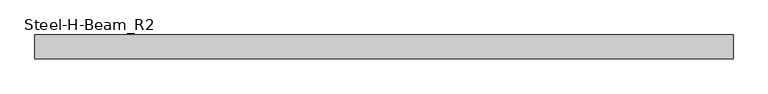
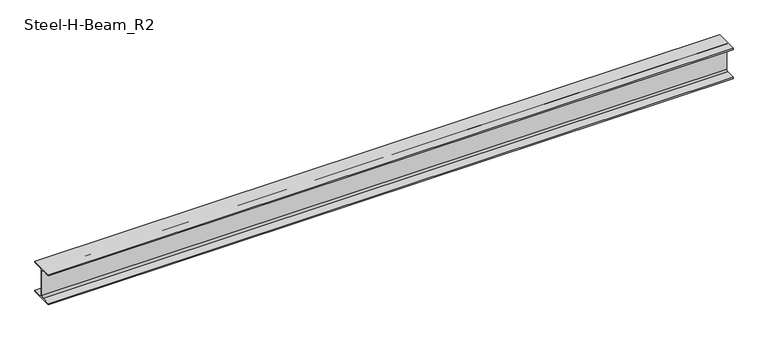
"""IFC4 building model written with IfcOpenShell, lengths in millimetres: beam geometry, Steel-H-Beam_R2 : BM121_H-340×250x9x14_SG1."""

from ifc_helpers import new_model, si_unit, point, frame, frame_2d, origin, place, context, project, spatial, polyline, circle_curve, trimmed, segment, composite_curve, outline, extrude, source, transform, mapped, element, save


def steel_h_beam_r2_7d9a1970(model_context):
    return source(origin(), model_context, "Body", "SweptSolid", [
        extrude(outline(composite_curve([segment(polyline([(125.0, -156.0), (125.0, -170.0), (-125.0, -170.0), (-125.0, -156.0), (-24.5, -156.0)]), True, "CONTINUOUS"), segment(trimmed(circle_curve(frame_2d((-24.5, -136.0)), 20.0), [point((-24.5, -156.0))], [point((-4.5, -136.0))], True, "CARTESIAN"), True, "CONTINUOUS"), segment(polyline([(-4.5, -136.0), (-4.5, 136.0)]), True, "CONTINUOUS"), segment(trimmed(circle_curve(frame_2d((-24.5, 136.0)), 20.0), [point((-4.5, 136.0))], [point((-24.5, 156.0))], True, "CARTESIAN"), True, "CONTINUOUS"), segment(polyline([(-24.5, 156.0), (-125.0, 156.0), (-125.0, 170.0), (125.0, 170.0), (125.0, 156.0), (24.5, 156.0)]), True, "CONTINUOUS"), segment(trimmed(circle_curve(frame_2d((24.5, 136.0)), 20.0), [point((24.5, 156.0))], [point((4.5, 136.0))], True, "CARTESIAN"), True, "CONTINUOUS"), segment(polyline([(4.5, 136.0), (4.5, -136.0)]), True, "CONTINUOUS"), segment(trimmed(circle_curve(frame_2d((24.5, -136.0)), 20.0), [point((4.5, -136.0))], [point((24.5, -156.0))], True, "CARTESIAN"), True, "CONTINUOUS"), segment(polyline([(24.5, -156.0), (125.0, -156.0)]), True, "CONTINUOUS")], self_intersect=False)), frame((-4287.3, 0.0, 0.0), z_axis=(1.0, 0.0, 0.0), x_axis=(0.0, 1.0, 0.0)), (0.0, 0.0, 1.0), 7287.3),
    ])


if __name__ == "__main__":
    model = new_model("IFC4")
    model_context = context("Model", 3, world=origin())
    ifc_project = project(units=[si_unit("LENGTHUNIT", "METRE", prefix="MILLI")], contexts=[model_context])
    site = spatial("IfcSite", under=ifc_project)
    building = spatial("IfcBuilding", under=site)
    placement = place(None, origin())
    steel_h_beam_r2_shape = steel_h_beam_r2_7d9a1970(model_context)
    element("IfcBeam", 1, ObjectType="Steel-H-Beam_R2 : BM121_H-340×250x9x14_SG1", at=placement, inside=building, context=model_context, shape_type="MappedRepresentation", body=[
        mapped(steel_h_beam_r2_shape, transform((0.0, 0.0, 0.0), x_axis=(1.0, 0.0, 0.0), y_axis=(0.0, 1.0, 0.0), z_axis=(0.0, 0.0, 1.0))),
    ])
    save(model, "model.ifc")

# Revit data of these elements
# Type "Steel-H-Beam_R2 : BM121_H-340×250x9x14_SG1"
#   SteelWeight = "Medium"
#   Surface Area = 1.62766 m²/m
#   Section Area = 101.514 cm²
#   Mass per Unit Length = 79.6882 kg/m
#   Length [instance default] = 3000 mm
#   B = 250 mm
#   H = 340 mm
#   r = 20 mm
#   tw = 9 mm
#   tf = 14 mm
#   hec_material4 [instance default] = none
#   hec_material3 [instance default] = none
#   hec_material2 [instance default] = none
#   hec_material1 [instance default] = none
#   Structural Material [instance default] = Steel, 45-345
#   Assembly Code = ""
# Element 1 (IfcBeam, "Steel-H-Beam_R2 : BM121_H-340×250x9x14_SG1")
#   Materials on its faces: "Steel, 45-345"
# Materials
#   "Steel, 45-345": class "Metal", colour RGB 189 187 185, transparency 0, Description = "Steel 345 MPa", Cost = 0
